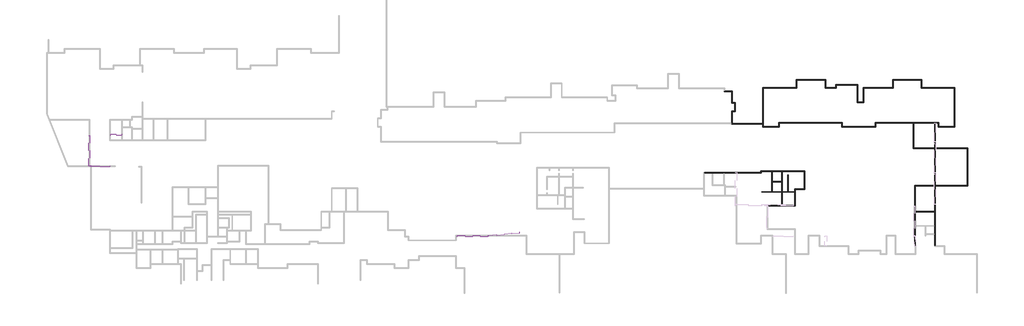
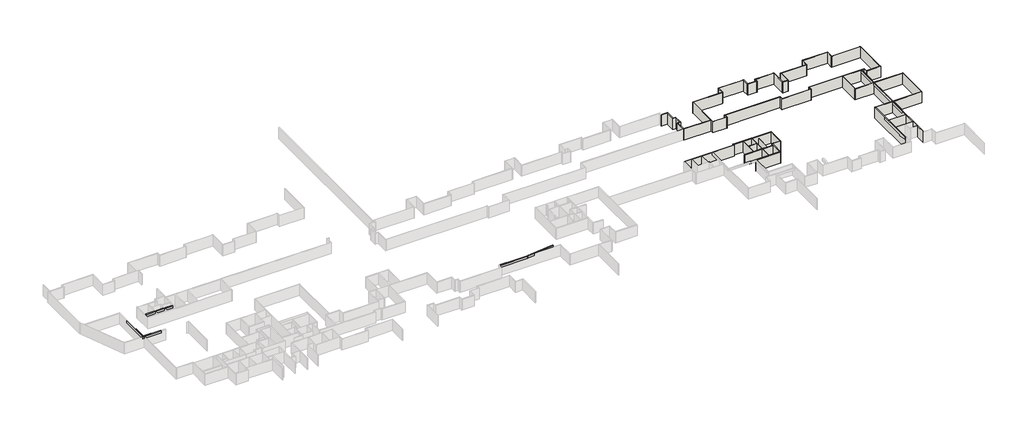
# One storey, part 7 of 8: 55 walls, 5 beams.
"""IFC4 building model written with IfcOpenShell, lengths in millimetres."""

from ifc_helpers import new_model, si_unit, frame, origin, origin_with_axes, place, context, project, spatial, polyline, outline, extrude, faceted_brep, element, save

model = new_model("IFC4")

# Units and contexts
model_context = context("Model", 3, world=origin())
ifc_project = project(units=[si_unit("LENGTHUNIT", "METRE", prefix="MILLI")], contexts=[model_context])

# Site, building, storey
site = spatial("IfcSite", under=ifc_project)
building = spatial("IfcBuilding", under=site)
storey = spatial("IfcBuildingStorey", under=building, Name="户型图", Elevation=0.0)

# Beams
placement = place(None, origin())
element("IfcBeam", 1, ObjectType="混凝土 - 矩形梁 : KL_beam", at=placement, inside=storey, context=model_context, shape_type="Brep", body=[
    faceted_brep([(96423.8477403, 45092.6668088, 3300.0), (96723.8477403, 45092.6668088, 3300.0), (96723.8477403, 45182.6668088, 3300.0), (96723.8477403, 52816.9449825, 3300.0), (96466.2302805, 52816.9449825, 3300.0), (96423.8477403, 52816.9449825, 3300.0), (96423.8477403, 45092.6668088, 2700.0), (96423.8477403, 52816.9449825, 2700.0), (96723.8477403, 45092.6668088, 2700.0), (96466.2302805, 52816.9449825, 2700.0), (96723.8477403, 52816.9449825, 2700.0), (96723.8477403, 45182.6668088, 2700.0)], [[[0, 1, 2, 3, 4, 5]], [[6, 0, 5, 7]], [[8, 6, 7, 9, 10, 11]], [[1, 8, 11, 10, 3, 2]], [[1, 0, 6, 8]], [[3, 10, 9, 7, 5, 4]]]),
])
element("IfcBeam", 2, ObjectType="混凝土 - 矩形梁 : KL_beam", at=placement, inside=storey, context=model_context, shape_type="Brep", body=[
    faceted_brep([(96423.8477403, 44972.6668088, 3300.0), (96423.8477403, 44882.6668088, 3300.0), (96858.261361, 44882.6668088, 3300.0), (96858.261361, 44972.6668088, 3300.0), (96423.8477403, 44882.6668088, 2700.0), (96423.8477403, 44972.6668088, 2700.0), (96858.261361, 44972.6668088, 2700.0), (96858.261361, 44882.6668088, 2700.0)], [[[0, 1, 2, 3]], [[4, 5, 6, 7]], [[1, 4, 7, 2]], [[4, 1, 0, 5]], [[5, 0, 3, 6]], [[3, 2, 7, 6]]]),
    faceted_brep([(101648.7128309, 45182.6668088, 3300.0), (101648.7128309, 45182.6668088, 2700.0), (96723.8477403, 45182.6668088, 2700.0), (96723.8477403, 45182.6668088, 3300.0), (101648.7128309, 44882.6668088, 3300.0), (101648.7128309, 44882.6668088, 2700.0), (96723.8477403, 45092.6668088, 2700.0), (96723.8477403, 45092.6668088, 3300.0), (96978.261361, 45092.6668088, 2700.0), (96978.261361, 45092.6668088, 3300.0), (96978.261361, 44882.6668088, 2700.0), (96978.261361, 44882.6668088, 3300.0), (96978.261361, 44972.6668088, 3300.0)], [[[0, 1, 2, 3]], [[0, 4, 5, 1]], [[3, 2, 6, 7]], [[8, 9, 7, 6]], [[9, 8, 10, 11, 12]], [[4, 0, 3, 7, 9, 12, 11]], [[1, 5, 10, 8, 6, 2]], [[5, 4, 11, 10]]]),
])
element("IfcBeam", 3, ObjectType="混凝土 - 矩形梁 : KL_beam", at=placement, inside=storey, context=model_context, shape_type="SweptSolid", body=[
    extrude(outline(polyline([(188793.7845861, 27383.0583741), (188793.7845861, 27683.0583741), (196393.7845861, 27683.0583741), (196393.7845861, 27536.9862623), (196385.7175673, 27383.0583741), (188793.7845861, 27383.0583741)])), frame((0.0, 0.0, 2700.0), z_axis=(0.0, 0.0, 1.0), x_axis=(1.0, 0.0, 0.0)), (0.0, 0.0, 1.0), 600.0),
])
element("IfcBeam", 4, ObjectType="混凝土 - 矩形梁 : KL_beam", at=placement, inside=storey, context=model_context, shape_type="Brep", body=[
    faceted_brep([(196693.7845861, 27529.1304858, 3300.0), (196686.9330908, 27398.3961679, 3300.0), (204278.3545725, 28263.2416532, 3300.0), (204280.088311, 28283.0583741, 3300.0), (204293.7845861, 28439.6075155, 3300.0), (204293.7845861, 28566.9400301, 3300.0), (196693.7845861, 27701.1172453, 3300.0), (196693.7845861, 27683.0583741, 3300.0), (196686.9330908, 27398.3961679, 2700.0), (204278.3545725, 28263.2416532, 2700.0), (196693.7845861, 27529.1304858, 2700.0), (196693.7845861, 27683.0583741, 2700.0), (196693.7845861, 27701.1172453, 2700.0), (204293.7845861, 28566.9400301, 2700.0), (204293.7845861, 28439.6075155, 2700.0), (204280.088311, 28283.0583741, 2700.0)], [[[0, 1, 2, 3, 4, 5, 6, 7]], [[1, 8, 9, 2]], [[8, 10, 11, 12, 13, 14, 15, 9]], [[12, 6, 5, 13]], [[6, 12, 11, 10, 0, 7]], [[1, 0, 10, 8]], [[5, 4, 14, 13]], [[2, 9, 15, 14, 4, 3]]]),
])
element("IfcBeam", 5, ObjectType="混凝土 - 矩形梁 : KL_beam", at=placement, inside=storey, context=model_context, shape_type="Brep", body=[
    faceted_brep([(109598.8477351, 52816.9449825, 3300.0), (109598.8477351, 53082.6668088, 3300.0), (109598.8477351, 53116.9449825, 3300.0), (107358.8477337, 53116.9449825, 3300.0), (107358.8477337, 52816.9449825, 3300.0), (109598.8477351, 52816.9449825, 2700.0), (107358.8477337, 52816.9449825, 2700.0), (109598.8477351, 53116.9449825, 2700.0), (109598.8477351, 53082.6668088, 2700.0), (107358.8477337, 53116.9449825, 2700.0)], [[[0, 1, 2, 3, 4]], [[5, 0, 4, 6]], [[7, 8, 5, 6, 9]], [[2, 7, 9, 3]], [[0, 5, 8, 7, 2, 1]], [[4, 3, 9, 6]]]),
    faceted_brep([(101948.7128309, 52816.9449825, 3300.0), (101948.7128309, 53116.9449825, 3300.0), (101948.7128309, 53116.9449825, 2700.0), (101948.7128309, 52816.9449825, 2700.0), (104655.6151291, 53116.9449825, 3300.0), (104655.6151291, 52816.9449825, 3300.0), (104655.6151291, 52816.9449825, 2700.0), (104655.6151291, 53116.9449825, 2700.0)], [[[0, 1, 2, 3]], [[4, 5, 6, 7]], [[1, 0, 5, 4]], [[0, 3, 6, 5]], [[3, 2, 7, 6]], [[2, 1, 4, 7]]]),
    faceted_brep([(104775.6151291, 52816.9449825, 3300.0), (104775.6151291, 53116.9449825, 3300.0), (104775.6151291, 53116.9449825, 2700.0), (104775.6151291, 52816.9449825, 2700.0), (107238.8477337, 53116.9449825, 3300.0), (107238.8477337, 52816.9449825, 3300.0), (107238.8477337, 52816.9449825, 2700.0), (107238.8477337, 53116.9449825, 2700.0)], [[[0, 1, 2, 3]], [[4, 5, 6, 7]], [[1, 0, 5, 4]], [[0, 3, 6, 5]], [[3, 2, 7, 6]], [[2, 1, 4, 7]]]),
])

# Walls
element("IfcWall", 6, ObjectType="所有墙体", at=placement, inside=storey, context=model_context, shape_type="Brep", body=[
    faceted_brep([(308483.5691593, 25066.2785565, 0.0), (308483.5691593, 40156.649759, 0.0), (308483.5691593, 40156.649759, 3300.0), (308483.5691593, 25066.2785565, 3300.0), (308363.5691593, 25066.2785565, 0.0), (308363.5691593, 25066.2785565, 3300.0), (308363.5691593, 27981.6313737, 3300.0), (308363.5691593, 28101.6313737, 3300.0), (308363.5691593, 30029.7325058, 3300.0), (308363.5691593, 30149.7325058, 3300.0), (308363.5691593, 33606.8475615, 3300.0), (308363.5691593, 33726.8475615, 3300.0), (308363.5691593, 40156.649759, 3300.0), (308363.5691593, 40156.649759, 0.0), (308363.5691593, 33726.8475615, 0.0), (308363.5691593, 33606.8475615, 0.0), (308363.5691593, 30149.7325058, 0.0), (308363.5691593, 30029.7325058, 0.0), (308363.5691593, 28101.6313737, 0.0), (308363.5691593, 27981.6313737, 0.0)], [[[0, 1, 2, 3]], [[4, 5, 6, 7, 8, 9, 10, 11, 12, 13, 14, 15, 16, 17, 18, 19]], [[1, 0, 4, 19, 18, 17, 16, 15, 14, 13]], [[3, 2, 12, 11, 10, 9, 8, 7, 6, 5]], [[0, 3, 5, 4]], [[2, 1, 13, 12]]]),
])
element("IfcWall", 7, ObjectType="所有墙体", at=placement, inside=storey, context=model_context, shape_type="Brep", body=[
    faceted_brep([(303458.8473874, 40156.649759, 0.0), (308363.5691593, 40156.649759, 0.0), (308483.5691593, 40156.649759, 0.0), (316708.8239545, 40156.649759, 0.0), (316708.8239545, 40156.649759, 3300.0), (308483.5691593, 40156.649759, 3300.0), (308363.5691593, 40156.649759, 3300.0), (303458.8473874, 40156.649759, 3300.0), (303458.8473874, 40276.649759, 0.0), (303458.8473874, 40276.649759, 3300.0), (308363.5691593, 40276.649759, 3300.0), (308483.5691593, 40276.649759, 3300.0), (316588.8239545, 40276.649759, 3300.0), (316708.8239545, 40276.649759, 3300.0), (316708.8239545, 40276.649759, 0.0), (316588.8239545, 40276.649759, 0.0), (308483.5691593, 40276.649759, 0.0), (308363.5691593, 40276.649759, 0.0)], [[[0, 1, 2, 3, 4, 5, 6, 7]], [[8, 9, 10, 11, 12, 13, 14, 15, 16, 17]], [[3, 2, 1, 0, 8, 17, 16, 15, 14]], [[7, 6, 5, 4, 13, 12, 11, 10, 9]], [[4, 3, 14, 13]], [[0, 7, 9, 8]]]),
])
element("IfcWall", 8, ObjectType="所有墙体", at=placement, inside=storey, context=model_context, shape_type="Brep", body=[
    faceted_brep([(316708.8239545, 40276.649759, 0.0), (316708.8239545, 49676.9053712, 0.0), (316708.8239545, 49676.9053712, 3300.0), (316708.8239545, 40276.649759, 3300.0), (316588.8239545, 40276.649759, 0.0), (316588.8239545, 40276.649759, 3300.0), (316588.8239545, 49556.9053712, 3300.0), (316588.8239545, 49676.9053712, 3300.0), (316588.8239545, 49676.9053712, 0.0), (316588.8239545, 49556.9053712, 0.0)], [[[0, 1, 2, 3]], [[4, 5, 6, 7, 8, 9]], [[1, 0, 4, 9, 8]], [[3, 2, 7, 6, 5]], [[0, 3, 5, 4]], [[2, 1, 8, 7]]]),
])
element("IfcWall", 9, ObjectType="所有墙体", at=placement, inside=storey, context=model_context, shape_type="SweptSolid", body=[
    extrude(outline(polyline([(308483.5691593, 49676.9053712), (316588.8239545, 49676.9053712), (316588.8239545, 49556.9053712), (308483.5691593, 49556.9053712), (308483.5691593, 49676.9053712)])), origin_with_axes(), (0.0, 0.0, 1.0), 3300.0),
])
element("IfcWall", 10, ObjectType="所有墙体", at=placement, inside=storey, context=model_context, shape_type="Brep", body=[
    faceted_brep([(308483.5691593, 40276.649759, 0.0), (308483.5691593, 49556.9053712, 0.0), (308483.5691593, 49676.9053712, 0.0), (308483.5691593, 55854.3583824, 0.0), (308483.5691593, 55854.3583824, 3300.0), (308483.5691593, 49676.9053712, 3300.0), (308483.5691593, 49556.9053712, 3300.0), (308483.5691593, 40276.649759, 3300.0), (308363.5691593, 40276.649759, 0.0), (308363.5691593, 40276.649759, 3300.0), (308363.5691593, 49556.9053712, 3300.0), (308363.5691593, 49676.9053712, 3300.0), (308363.5691593, 55854.3583824, 3300.0), (308363.5691593, 55854.3583824, 0.0), (308363.5691593, 49676.9053712, 0.0), (308363.5691593, 49556.9053712, 0.0)], [[[0, 1, 2, 3, 4, 5, 6, 7]], [[8, 9, 10, 11, 12, 13, 14, 15]], [[3, 2, 1, 0, 8, 15, 14, 13]], [[7, 6, 5, 4, 12, 11, 10, 9]], [[4, 3, 13, 12]], [[0, 7, 9, 8]]]),
])
element("IfcWall", 11, ObjectType="所有墙体", at=placement, inside=storey, context=model_context, shape_type="Brep", body=[
    faceted_brep([(293431.9735661, 55854.3583824, 0.0), (293551.9735661, 55854.3583824, 0.0), (302988.8797699, 55854.3583824, 0.0), (303108.8797699, 55854.3583824, 0.0), (308363.5691593, 55854.3583824, 0.0), (308483.5691593, 55854.3583824, 0.0), (309231.9735597, 55854.3583824, 0.0), (309351.9735597, 55854.3583824, 0.0), (309351.9735597, 55854.3583824, 3300.0), (309231.9735597, 55854.3583824, 3300.0), (308483.5691593, 55854.3583824, 3300.0), (308363.5691593, 55854.3583824, 3300.0), (303108.8797699, 55854.3583824, 3300.0), (302988.8797699, 55854.3583824, 3300.0), (293551.9735661, 55854.3583824, 3300.0), (293431.9735661, 55854.3583824, 3300.0), (293431.9735661, 55974.3583824, 0.0), (293431.9735661, 55974.3583824, 3300.0), (309351.9735597, 55974.3583824, 3300.0), (309351.9735597, 55974.3583824, 0.0)], [[[0, 1, 2, 3, 4, 5, 6, 7, 8, 9, 10, 11, 12, 13, 14, 15]], [[16, 17, 18, 19]], [[7, 6, 5, 4, 3, 2, 1, 0, 16, 19]], [[15, 14, 13, 12, 11, 10, 9, 8, 18, 17]], [[8, 7, 19, 18]], [[0, 15, 17, 16]]]),
])
element("IfcWall", 12, ObjectType="所有墙体", at=placement, inside=storey, context=model_context, shape_type="Brep", body=[
    faceted_brep([(309231.9735597, 55854.3583824, 0.0), (309231.9735597, 54854.3583848, 0.0), (309231.9735597, 54854.3583848, 3300.0), (309231.9735597, 55854.3583824, 3300.0), (309351.9735597, 55854.3583824, 0.0), (309351.9735597, 55854.3583824, 3300.0), (309351.9735597, 54974.3583848, 3300.0), (309351.9735597, 54854.3583848, 3300.0), (309351.9735597, 54854.3583848, 0.0), (309351.9735597, 54974.3583848, 0.0)], [[[0, 1, 2, 3]], [[4, 5, 6, 7, 8, 9]], [[1, 0, 4, 9, 8]], [[3, 2, 7, 6, 5]], [[0, 3, 5, 4]], [[2, 1, 8, 7]]]),
])
element("IfcWall", 13, ObjectType="所有墙体", at=placement, inside=storey, context=model_context, shape_type="Brep", body=[
    faceted_brep([(309351.9735597, 54854.3583848, 0.0), (313351.9735669, 54854.3583848, 0.0), (313351.9735669, 54854.3583848, 3300.0), (309351.9735597, 54854.3583848, 3300.0), (309351.9735597, 54974.3583848, 0.0), (309351.9735597, 54974.3583848, 3300.0), (313231.9735669, 54974.3583848, 3300.0), (313351.9735669, 54974.3583848, 3300.0), (313351.9735669, 54974.3583848, 0.0), (313231.9735669, 54974.3583848, 0.0)], [[[0, 1, 2, 3]], [[4, 5, 6, 7, 8, 9]], [[1, 0, 4, 9, 8]], [[3, 2, 7, 6, 5]], [[0, 3, 5, 4]], [[2, 1, 8, 7]]]),
])
element("IfcWall", 14, ObjectType="所有墙体", at=placement, inside=storey, context=model_context, shape_type="Brep", body=[
    faceted_brep([(313351.9735669, 54974.3583848, 0.0), (313351.9735669, 64774.3583829, 0.0), (313351.9735669, 64774.3583829, 3300.0), (313351.9735669, 54974.3583848, 3300.0), (313231.9735669, 54974.3583848, 0.0), (313231.9735669, 54974.3583848, 3300.0), (313231.9735669, 64654.3583829, 3300.0), (313231.9735669, 64774.3583829, 3300.0), (313231.9735669, 64774.3583829, 0.0), (313231.9735669, 64654.3583829, 0.0)], [[[0, 1, 2, 3]], [[4, 5, 6, 7, 8, 9]], [[1, 0, 4, 9, 8]], [[3, 2, 7, 6, 5]], [[0, 3, 5, 4]], [[2, 1, 8, 7]]]),
])
element("IfcWall", 15, ObjectType="所有墙体", at=placement, inside=storey, context=model_context, shape_type="Brep", body=[
    faceted_brep([(313231.9735669, 64774.3583829, 0.0), (305151.9735626, 64774.3583829, 0.0), (305031.9735626, 64774.3583829, 0.0), (305031.9735626, 64774.3583829, 3300.0), (305151.9735626, 64774.3583829, 3300.0), (313231.9735669, 64774.3583829, 3300.0), (313231.9735669, 64654.3583829, 0.0), (313231.9735669, 64654.3583829, 3300.0), (305031.9735626, 64654.3583829, 3300.0), (305031.9735626, 64654.3583829, 0.0)], [[[0, 1, 2, 3, 4, 5]], [[6, 7, 8, 9]], [[2, 1, 0, 6, 9]], [[5, 4, 3, 8, 7]], [[0, 5, 7, 6]], [[3, 2, 9, 8]]]),
])
element("IfcWall", 16, ObjectType="所有墙体", at=placement, inside=storey, context=model_context, shape_type="Brep", body=[
    faceted_brep([(305151.9735626, 64774.3583829, 0.0), (305151.9735626, 66774.3583864, 0.0), (305151.9735626, 66774.3583864, 3300.0), (305151.9735626, 64774.3583829, 3300.0), (305031.9735626, 64774.3583829, 0.0), (305031.9735626, 64774.3583829, 3300.0), (305031.9735626, 66654.3583864, 3300.0), (305031.9735626, 66774.3583864, 3300.0), (305031.9735626, 66774.3583864, 0.0), (305031.9735626, 66654.3583864, 0.0)], [[[0, 1, 2, 3]], [[4, 5, 6, 7, 8, 9]], [[1, 0, 4, 9, 8]], [[3, 2, 7, 6, 5]], [[0, 3, 5, 4]], [[2, 1, 8, 7]]]),
])
element("IfcWall", 17, ObjectType="所有墙体", at=placement, inside=storey, context=model_context, shape_type="Brep", body=[
    faceted_brep([(305031.9735626, 66774.3583864, 0.0), (297831.9735583, 66774.3583864, 0.0), (297831.9735583, 66774.3583864, 3300.0), (305031.9735626, 66774.3583864, 3300.0), (305031.9735626, 66654.3583864, 0.0), (305031.9735626, 66654.3583864, 3300.0), (297951.9735583, 66654.3583864, 3300.0), (297831.9735583, 66654.3583864, 3300.0), (297831.9735583, 66654.3583864, 0.0), (297951.9735583, 66654.3583864, 0.0)], [[[0, 1, 2, 3]], [[4, 5, 6, 7, 8, 9]], [[1, 0, 4, 9, 8]], [[3, 2, 7, 6, 5]], [[0, 3, 5, 4]], [[2, 1, 8, 7]]]),
])
element("IfcWall", 18, ObjectType="所有墙体", at=placement, inside=storey, context=model_context, shape_type="Brep", body=[
    faceted_brep([(297831.9735583, 66654.3583864, 0.0), (297831.9735583, 64774.3583829, 0.0), (297831.9735583, 64654.3583829, 0.0), (297831.9735583, 64654.3583829, 3300.0), (297831.9735583, 64774.3583829, 3300.0), (297831.9735583, 66654.3583864, 3300.0), (297951.9735583, 66654.3583864, 0.0), (297951.9735583, 66654.3583864, 3300.0), (297951.9735583, 64654.3583829, 3300.0), (297951.9735583, 64654.3583829, 0.0)], [[[0, 1, 2, 3, 4, 5]], [[6, 7, 8, 9]], [[2, 1, 0, 6, 9]], [[5, 4, 3, 8, 7]], [[0, 5, 7, 6]], [[3, 2, 9, 8]]]),
])
element("IfcWall", 19, ObjectType="所有墙体", at=placement, inside=storey, context=model_context, shape_type="Brep", body=[
    faceted_brep([(297831.9735583, 64774.3583829, 0.0), (290431.9735626, 64774.3583829, 0.0), (290431.9735626, 64774.3583829, 3300.0), (297831.9735583, 64774.3583829, 3300.0), (297831.9735583, 64654.3583829, 0.0), (297831.9735583, 64654.3583829, 3300.0), (290551.9735626, 64654.3583829, 3300.0), (290431.9735626, 64654.3583829, 3300.0), (290431.9735626, 64654.3583829, 0.0), (290551.9735626, 64654.3583829, 0.0)], [[[0, 1, 2, 3]], [[4, 5, 6, 7, 8, 9]], [[1, 0, 4, 9, 8]], [[3, 2, 7, 6, 5]], [[0, 3, 5, 4]], [[2, 1, 8, 7]]]),
])
element("IfcWall", 20, ObjectType="所有墙体", at=placement, inside=storey, context=model_context, shape_type="Brep", body=[
    faceted_brep([(290431.9735626, 64654.3583829, 0.0), (290431.9735626, 61174.3583823, 0.0), (290431.9735626, 61054.3583823, 0.0), (290431.9735626, 61054.3583823, 3300.0), (290431.9735626, 61174.3583823, 3300.0), (290431.9735626, 64654.3583829, 3300.0), (290551.9735626, 64654.3583829, 0.0), (290551.9735626, 64654.3583829, 3300.0), (290551.9735626, 61054.3583823, 3300.0), (290551.9735626, 61054.3583823, 0.0)], [[[0, 1, 2, 3, 4, 5]], [[6, 7, 8, 9]], [[2, 1, 0, 6, 9]], [[5, 4, 3, 8, 7]], [[0, 5, 7, 6]], [[3, 2, 9, 8]]]),
])
element("IfcWall", 21, ObjectType="所有墙体", at=placement, inside=storey, context=model_context, shape_type="Brep", body=[
    faceted_brep([(290431.9735626, 61174.3583823, 0.0), (289051.9735625, 61174.3583823, 0.0), (288931.9735625, 61174.3583823, 0.0), (288931.9735625, 61174.3583823, 3300.0), (289051.9735625, 61174.3583823, 3300.0), (290431.9735626, 61174.3583823, 3300.0), (290431.9735626, 61054.3583823, 0.0), (290431.9735626, 61054.3583823, 3300.0), (288931.9735625, 61054.3583823, 3300.0), (288931.9735625, 61054.3583823, 0.0)], [[[0, 1, 2, 3, 4, 5]], [[6, 7, 8, 9]], [[2, 1, 0, 6, 9]], [[5, 4, 3, 8, 7]], [[0, 5, 7, 6]], [[3, 2, 9, 8]]]),
])
element("IfcWall", 22, ObjectType="所有墙体", at=placement, inside=storey, context=model_context, shape_type="Brep", body=[
    faceted_brep([(289051.9735625, 61174.3583823, 0.0), (289051.9735625, 65574.3800091, 0.0), (289051.9735625, 65574.3800091, 3300.0), (289051.9735625, 61174.3583823, 3300.0), (288931.9735625, 61174.3583823, 0.0), (288931.9735625, 61174.3583823, 3300.0), (288931.9735625, 65454.3800091, 3300.0), (288931.9735625, 65574.3800091, 3300.0), (288931.9735625, 65574.3800091, 0.0), (288931.9735625, 65454.3800091, 0.0)], [[[0, 1, 2, 3]], [[4, 5, 6, 7, 8, 9]], [[1, 0, 4, 9, 8]], [[3, 2, 7, 6, 5]], [[0, 3, 5, 4]], [[2, 1, 8, 7]]]),
])
element("IfcWall", 23, ObjectType="所有墙体", at=placement, inside=storey, context=model_context, shape_type="Brep", body=[
    faceted_brep([(288931.9735625, 65574.3800091, 0.0), (283531.9735562, 65574.3800091, 0.0), (283531.9735562, 65574.3800091, 3300.0), (288931.9735625, 65574.3800091, 3300.0), (288931.9735625, 65454.3800091, 0.0), (288931.9735625, 65454.3800091, 3300.0), (283651.9735562, 65454.3800091, 3300.0), (283531.9735562, 65454.3800091, 3300.0), (283531.9735562, 65454.3800091, 0.0), (283651.9735562, 65454.3800091, 0.0)], [[[0, 1, 2, 3]], [[4, 5, 6, 7, 8, 9]], [[1, 0, 4, 9, 8]], [[3, 2, 7, 6, 5]], [[0, 3, 5, 4]], [[2, 1, 8, 7]]]),
])
element("IfcWall", 24, ObjectType="所有墙体", at=placement, inside=storey, context=model_context, shape_type="Brep", body=[
    faceted_brep([(283531.9735562, 65454.3800091, 0.0), (283531.9735562, 64774.3583829, 0.0), (283531.9735562, 64654.3583829, 0.0), (283531.9735562, 64654.3583829, 3300.0), (283531.9735562, 64774.3583829, 3300.0), (283531.9735562, 65454.3800091, 3300.0), (283651.9735562, 65454.3800091, 0.0), (283651.9735562, 65454.3800091, 3300.0), (283651.9735562, 64654.3583829, 3300.0), (283651.9735562, 64654.3583829, 0.0)], [[[0, 1, 2, 3, 4, 5]], [[6, 7, 8, 9]], [[2, 1, 0, 6, 9]], [[5, 4, 3, 8, 7]], [[0, 5, 7, 6]], [[3, 2, 9, 8]]]),
])
element("IfcWall", 25, ObjectType="所有墙体", at=placement, inside=storey, context=model_context, shape_type="Brep", body=[
    faceted_brep([(283531.9735562, 64774.3583829, 0.0), (281051.9735665, 64774.3583829, 0.0), (280931.9735665, 64774.3583829, 0.0), (280931.9735665, 64774.3583829, 3300.0), (281051.9735665, 64774.3583829, 3300.0), (283531.9735562, 64774.3583829, 3300.0), (283531.9735562, 64654.3583829, 0.0), (283531.9735562, 64654.3583829, 3300.0), (280931.9735665, 64654.3583829, 3300.0), (280931.9735665, 64654.3583829, 0.0)], [[[0, 1, 2, 3, 4, 5]], [[6, 7, 8, 9]], [[2, 1, 0, 6, 9]], [[5, 4, 3, 8, 7]], [[0, 5, 7, 6]], [[3, 2, 9, 8]]]),
])
element("IfcWall", 26, ObjectType="所有墙体", at=placement, inside=storey, context=model_context, shape_type="Brep", body=[
    faceted_brep([(281051.9735665, 64774.3583829, 0.0), (281051.9735665, 66774.3583864, 0.0), (281051.9735665, 66774.3583864, 3300.0), (281051.9735665, 64774.3583829, 3300.0), (280931.9735665, 64774.3583829, 0.0), (280931.9735665, 64774.3583829, 3300.0), (280931.9735665, 66654.3583864, 3300.0), (280931.9735665, 66774.3583864, 3300.0), (280931.9735665, 66774.3583864, 0.0), (280931.9735665, 66654.3583864, 0.0)], [[[0, 1, 2, 3]], [[4, 5, 6, 7, 8, 9]], [[1, 0, 4, 9, 8]], [[3, 2, 7, 6, 5]], [[0, 3, 5, 4]], [[2, 1, 8, 7]]]),
])
element("IfcWall", 27, ObjectType="所有墙体", at=placement, inside=storey, context=model_context, shape_type="Brep", body=[
    faceted_brep([(280931.9735665, 66774.3583864, 0.0), (273731.9735661, 66774.3583864, 0.0), (273731.9735661, 66774.3583864, 3300.0), (280931.9735665, 66774.3583864, 3300.0), (280931.9735665, 66654.3583864, 0.0), (280931.9735665, 66654.3583864, 3300.0), (273851.9735661, 66654.3583864, 3300.0), (273731.9735661, 66654.3583864, 3300.0), (273731.9735661, 66654.3583864, 0.0), (273851.9735661, 66654.3583864, 0.0)], [[[0, 1, 2, 3]], [[4, 5, 6, 7, 8, 9]], [[1, 0, 4, 9, 8]], [[3, 2, 7, 6, 5]], [[0, 3, 5, 4]], [[2, 1, 8, 7]]]),
])
element("IfcWall", 28, ObjectType="所有墙体", at=placement, inside=storey, context=model_context, shape_type="Brep", body=[
    faceted_brep([(273731.9735661, 66654.3583864, 0.0), (273731.9735661, 64774.3583829, 0.0), (273731.9735661, 64654.3583829, 0.0), (273731.9735661, 64654.3583829, 3300.0), (273731.9735661, 64774.3583829, 3300.0), (273731.9735661, 66654.3583864, 3300.0), (273851.9735661, 66654.3583864, 0.0), (273851.9735661, 66654.3583864, 3300.0), (273851.9735661, 64654.3583829, 3300.0), (273851.9735661, 64654.3583829, 0.0)], [[[0, 1, 2, 3, 4, 5]], [[6, 7, 8, 9]], [[2, 1, 0, 6, 9]], [[5, 4, 3, 8, 7]], [[0, 5, 7, 6]], [[3, 2, 9, 8]]]),
])
element("IfcWall", 29, ObjectType="所有墙体", at=placement, inside=storey, context=model_context, shape_type="Brep", body=[
    faceted_brep([(273731.9735661, 64774.3583829, 0.0), (265331.9735637, 64774.3583829, 0.0), (265331.9735637, 64774.3583829, 3300.0), (273731.9735661, 64774.3583829, 3300.0), (273731.9735661, 64654.3583829, 0.0), (273731.9735661, 64654.3583829, 3300.0), (265451.9735637, 64654.3583829, 3300.0), (265331.9735637, 64654.3583829, 3300.0), (265331.9735637, 64654.3583829, 0.0), (265451.9735637, 64654.3583829, 0.0)], [[[0, 1, 2, 3]], [[4, 5, 6, 7, 8, 9]], [[1, 0, 4, 9, 8]], [[3, 2, 7, 6, 5]], [[0, 3, 5, 4]], [[2, 1, 8, 7]]]),
])
element("IfcWall", 30, ObjectType="所有墙体", at=placement, inside=storey, context=model_context, shape_type="Brep", body=[
    faceted_brep([(265331.9735637, 64654.3583829, 0.0), (265331.9735637, 55826.5251182, 0.0), (265331.9735637, 55706.5251182, 0.0), (265331.9735637, 54974.3583848, 0.0), (265331.9735637, 54974.3583848, 3300.0), (265331.9735637, 55706.5251182, 3300.0), (265331.9735637, 55826.5251182, 3300.0), (265331.9735637, 64654.3583829, 3300.0), (265451.9735637, 64654.3583829, 0.0), (265451.9735637, 64654.3583829, 3300.0), (265451.9735637, 54974.3583848, 3300.0), (265451.9735637, 54974.3583848, 0.0)], [[[0, 1, 2, 3, 4, 5, 6, 7]], [[8, 9, 10, 11]], [[3, 2, 1, 0, 8, 11]], [[7, 6, 5, 4, 10, 9]], [[0, 7, 9, 8]], [[4, 3, 11, 10]]]),
])
element("IfcWall", 31, ObjectType="所有墙体", at=placement, inside=storey, context=model_context, shape_type="Brep", body=[
    faceted_brep([(265331.9735637, 55826.5251182, 0.0), (257584.5015155, 55826.5251182, 0.0), (257464.5015155, 55826.5251182, 0.0), (257464.5015155, 55826.5251182, 3300.0), (257584.5015155, 55826.5251182, 3300.0), (265331.9735637, 55826.5251182, 3300.0), (265331.9735637, 55706.5251182, 0.0), (265331.9735637, 55706.5251182, 3300.0), (257464.5015155, 55706.5251182, 3300.0), (257464.5015155, 55706.5251182, 0.0), (257464.5015155, 55756.5110329, 0.0), (257464.5015155, 55756.5110329, 3300.0)], [[[0, 1, 2, 3, 4, 5]], [[6, 7, 8, 9]], [[2, 1, 0, 6, 9, 10]], [[5, 4, 3, 11, 8, 7]], [[0, 5, 7, 6]], [[3, 2, 10, 9, 8, 11]]]),
])
element("IfcWall", 32, ObjectType="所有墙体", at=placement, inside=storey, context=model_context, shape_type="Brep", body=[
    faceted_brep([(257584.5015155, 55826.5251182, 0.0), (257584.5015155, 58756.6395115, 0.0), (257584.5015155, 58876.6395115, 0.0), (257584.5015155, 58876.6395115, 3300.0), (257584.5015155, 58756.6395115, 3300.0), (257584.5015155, 55826.5251182, 3300.0), (257464.5015155, 55826.5251182, 0.0), (257464.5015155, 55826.5251182, 3300.0), (257464.5015155, 55876.5110329, 3300.0), (257464.5015155, 58876.6395115, 3300.0), (257464.5015155, 58876.6395115, 0.0), (257464.5015155, 55876.5110329, 0.0)], [[[0, 1, 2, 3, 4, 5]], [[6, 7, 8, 9, 10, 11]], [[2, 1, 0, 6, 11, 10]], [[5, 4, 3, 9, 8, 7]], [[0, 5, 7, 6]], [[3, 2, 10, 9]]]),
])
element("IfcWall", 33, ObjectType="所有墙体", at=placement, inside=storey, context=model_context, shape_type="Brep", body=[
    faceted_brep([(257584.5015155, 58756.6395115, 0.0), (258384.5015175, 58756.6395115, 0.0), (258384.5015175, 58756.6395115, 3300.0), (257584.5015155, 58756.6395115, 3300.0), (257584.5015155, 58876.6395115, 0.0), (257584.5015155, 58876.6395115, 3300.0), (258264.5015175, 58876.6395115, 3300.0), (258384.5015175, 58876.6395115, 3300.0), (258384.5015175, 58876.6395115, 0.0), (258264.5015175, 58876.6395115, 0.0)], [[[0, 1, 2, 3]], [[4, 5, 6, 7, 8, 9]], [[1, 0, 4, 9, 8]], [[3, 2, 7, 6, 5]], [[0, 3, 5, 4]], [[2, 1, 8, 7]]]),
])
element("IfcWall", 34, ObjectType="所有墙体", at=placement, inside=storey, context=model_context, shape_type="Brep", body=[
    faceted_brep([(258384.5015175, 58876.6395115, 0.0), (258384.5015175, 61076.6395927, 0.0), (258384.5015175, 61076.6395927, 3300.0), (258384.5015175, 58876.6395115, 3300.0), (258264.5015175, 58876.6395115, 0.0), (258264.5015175, 58876.6395115, 3300.0), (258264.5015175, 60956.6395927, 3300.0), (258264.5015175, 61076.6395927, 3300.0), (258264.5015175, 61076.6395927, 0.0), (258264.5015175, 60956.6395927, 0.0)], [[[0, 1, 2, 3]], [[4, 5, 6, 7, 8, 9]], [[1, 0, 4, 9, 8]], [[3, 2, 7, 6, 5]], [[0, 3, 5, 4]], [[2, 1, 8, 7]]]),
])
element("IfcWall", 35, ObjectType="所有墙体", at=placement, inside=storey, context=model_context, shape_type="Brep", body=[
    faceted_brep([(258264.5015175, 61076.6395927, 0.0), (257584.5015155, 61076.6395927, 0.0), (257464.5015155, 61076.6395927, 0.0), (257464.5015155, 61076.6395927, 3300.0), (257584.5015155, 61076.6395927, 3300.0), (258264.5015175, 61076.6395927, 3300.0), (258264.5015175, 60956.6395927, 0.0), (258264.5015175, 60956.6395927, 3300.0), (257464.5015155, 60956.6395927, 3300.0), (257464.5015155, 60956.6395927, 0.0)], [[[0, 1, 2, 3, 4, 5]], [[6, 7, 8, 9]], [[2, 1, 0, 6, 9]], [[5, 4, 3, 8, 7]], [[0, 5, 7, 6]], [[3, 2, 9, 8]]]),
])
element("IfcWall", 36, ObjectType="所有墙体", at=placement, inside=storey, context=model_context, shape_type="Brep", body=[
    faceted_brep([(257584.5015155, 61076.6395927, 0.0), (257584.5015155, 63876.5127734, 0.0), (257584.5015155, 63876.5127734, 3300.0), (257584.5015155, 61076.6395927, 3300.0), (257464.5015155, 61076.6395927, 0.0), (257464.5015155, 61076.6395927, 3300.0), (257464.5015155, 63756.5127734, 3300.0), (257464.5015155, 63876.5127734, 3300.0), (257464.5015155, 63876.5127734, 0.0), (257464.5015155, 63756.5127734, 0.0)], [[[0, 1, 2, 3]], [[4, 5, 6, 7, 8, 9]], [[1, 0, 4, 9, 8]], [[3, 2, 7, 6, 5]], [[0, 3, 5, 4]], [[2, 1, 8, 7]]]),
])
element("IfcWall", 37, ObjectType="所有墙体", at=placement, inside=storey, context=model_context, shape_type="Brep", body=[
    faceted_brep([(257464.5015155, 63876.5127734, 0.0), (255784.4931741, 63876.5127734, 0.0), (255664.4931741, 63876.5127734, 0.0), (255664.4931741, 63876.5127734, 3300.0), (255784.4931741, 63876.5127734, 3300.0), (257464.5015155, 63876.5127734, 3300.0), (257464.5015155, 63756.5127734, 0.0), (257464.5015155, 63756.5127734, 3300.0), (255664.4931741, 63756.5127734, 3300.0), (255664.4931741, 63756.5127734, 0.0)], [[[0, 1, 2, 3, 4, 5]], [[6, 7, 8, 9]], [[2, 1, 0, 6, 9]], [[5, 4, 3, 8, 7]], [[0, 5, 7, 6]], [[3, 2, 9, 8]]]),
])
element("IfcWall", 38, ObjectType="所有墙体", at=placement, inside=storey, context=model_context, shape_type="Brep", body=[
    faceted_brep([(250658.8239575, 43406.8473728, 0.0), (255513.6576827, 43406.8473728, 0.0), (255633.6576827, 43406.8473728, 0.0), (264932.3033606, 43406.8473728, 0.0), (264932.3033606, 43406.8473728, 3300.0), (255633.6576827, 43406.8473728, 3300.0), (255513.6576827, 43406.8473728, 3300.0), (250658.8239575, 43406.8473728, 3300.0), (250658.8239575, 43526.8473728, 0.0), (250658.8239575, 43526.8473728, 3300.0), (264812.3033606, 43526.8473728, 3300.0), (264932.3033606, 43526.8473728, 3300.0), (264932.3033606, 43526.8473728, 0.0), (264812.3033606, 43526.8473728, 0.0)], [[[0, 1, 2, 3, 4, 5, 6, 7]], [[8, 9, 10, 11, 12, 13]], [[3, 2, 1, 0, 8, 13, 12]], [[7, 6, 5, 4, 11, 10, 9]], [[0, 7, 9, 8]], [[4, 3, 12, 11]]]),
])
element("IfcWall", 39, ObjectType="所有墙体", at=placement, inside=storey, context=model_context, shape_type="Brep", body=[
    faceted_brep([(264932.3033606, 43526.8473728, 0.0), (264932.3033606, 43807.0754503, 0.0), (264932.3033606, 43927.0754503, 0.0), (264932.3033606, 43927.0754503, 3300.0), (264932.3033606, 43807.0754503, 3300.0), (264932.3033606, 43526.8473728, 3300.0), (264812.3033606, 43526.8473728, 0.0), (264812.3033606, 43526.8473728, 3300.0), (264812.3033606, 43927.0754503, 3300.0), (264812.3033606, 43927.0754503, 0.0)], [[[0, 1, 2, 3, 4, 5]], [[6, 7, 8, 9]], [[2, 1, 0, 6, 9]], [[5, 4, 3, 8, 7]], [[0, 5, 7, 6]], [[3, 2, 9, 8]]]),
])
element("IfcWall", 40, ObjectType="所有墙体", at=placement, inside=storey, context=model_context, shape_type="Brep", body=[
    faceted_brep([(264932.3033606, 43807.0754503, 0.0), (275663.8471108, 43807.0754503, 0.0), (275783.8471108, 43807.0754503, 0.0), (275783.8471108, 43807.0754503, 3300.0), (275663.8471108, 43807.0754503, 3300.0), (264932.3033606, 43807.0754503, 3300.0), (264932.3033606, 43927.0754503, 0.0), (264932.3033606, 43927.0754503, 3300.0), (275783.8471108, 43927.0754503, 3300.0), (275783.8471108, 43927.0754503, 0.0)], [[[0, 1, 2, 3, 4, 5]], [[6, 7, 8, 9]], [[2, 1, 0, 6, 9]], [[5, 4, 3, 8, 7]], [[0, 5, 7, 6]], [[3, 2, 9, 8]]]),
])
element("IfcWall", 41, ObjectType="所有墙体", at=placement, inside=storey, context=model_context, shape_type="Brep", body=[
    faceted_brep([(275663.8471108, 43807.0754503, 0.0), (275663.8471108, 39327.0768266, 0.0), (275663.8471108, 39207.0768266, 0.0), (275663.8471108, 39207.0768266, 3300.0), (275663.8471108, 39327.0768266, 3300.0), (275663.8471108, 43807.0754503, 3300.0), (275783.8471108, 43807.0754503, 0.0), (275783.8471108, 43807.0754503, 3300.0), (275783.8471108, 39207.0768266, 3300.0), (275783.8471108, 39207.0768266, 0.0)], [[[0, 1, 2, 3, 4, 5]], [[6, 7, 8, 9]], [[2, 1, 0, 6, 9]], [[5, 4, 3, 8, 7]], [[0, 5, 7, 6]], [[3, 2, 9, 8]]]),
])
element("IfcWall", 42, ObjectType="所有墙体", at=placement, inside=storey, context=model_context, shape_type="Brep", body=[
    faceted_brep([(275663.8471108, 39327.0768266, 0.0), (273288.1652502, 39327.0768266, 0.0), (273288.1652502, 39327.0768266, 3300.0), (275663.8471108, 39327.0768266, 3300.0), (275663.8471108, 39207.0768266, 0.0), (275663.8471108, 39207.0768266, 3300.0), (273408.1652502, 39207.0768266, 3300.0), (273288.1652502, 39207.0768266, 3300.0), (273288.1652502, 39207.0768266, 0.0), (273408.1652502, 39207.0768266, 0.0)], [[[0, 1, 2, 3]], [[4, 5, 6, 7, 8, 9]], [[1, 0, 4, 9, 8]], [[3, 2, 7, 6, 5]], [[0, 3, 5, 4]], [[2, 1, 8, 7]]]),
])
element("IfcWall", 43, ObjectType="所有墙体", at=placement, inside=storey, context=model_context, shape_type="Brep", body=[
    faceted_brep([(273288.1652502, 39207.0768266, 0.0), (273288.1652502, 35226.5508771, 0.0), (273288.1652502, 35106.5508771, 0.0), (273288.1652502, 35106.5508771, 3300.0), (273288.1652502, 35226.5508771, 3300.0), (273288.1652502, 39207.0768266, 3300.0), (273408.1652502, 39207.0768266, 0.0), (273408.1652502, 39207.0768266, 3300.0), (273408.1652502, 35106.5508771, 3300.0), (273408.1652502, 35106.5508771, 0.0)], [[[0, 1, 2, 3, 4, 5]], [[6, 7, 8, 9]], [[2, 1, 0, 6, 9]], [[5, 4, 3, 8, 7]], [[0, 5, 7, 6]], [[3, 2, 9, 8]]]),
])
element("IfcWall", 44, ObjectType="所有墙体", at=placement, inside=storey, context=model_context, shape_type="Brep", body=[
    faceted_brep([(273288.1652502, 35226.5508771, 0.0), (266363.353082, 35226.5508771, 0.0), (266363.353082, 35226.5508771, 3300.0), (273288.1652502, 35226.5508771, 3300.0), (273288.1652502, 35106.5508771, 0.0), (273288.1652502, 35106.5508771, 3300.0), (266483.353082, 35106.5508771, 3300.0), (266363.353082, 35106.5508771, 3300.0), (266363.353082, 35106.5508771, 0.0), (266483.353082, 35106.5508771, 0.0)], [[[0, 1, 2, 3]], [[4, 5, 6, 7, 8, 9]], [[1, 0, 4, 9, 8]], [[3, 2, 7, 6, 5]], [[0, 3, 5, 4]], [[2, 1, 8, 7]]]),
])
element("IfcWall", 45, ObjectType="所有墙体", at=placement, inside=storey, context=model_context, shape_type="Brep", body=[
    faceted_brep([(303458.8473874, 25067.4234213, 0.0), (303458.8473874, 30029.7325058, 0.0), (303458.8473874, 30149.7325058, 0.0), (303458.8473874, 33606.8475615, 0.0), (303458.8473874, 33726.8475615, 0.0), (303458.8473874, 40156.649759, 0.0), (303458.8473874, 40276.649759, 0.0), (303458.8473874, 40276.649759, 3300.0), (303458.8473874, 40156.649759, 3300.0), (303458.8473874, 33726.8475615, 3300.0), (303458.8473874, 33606.8475615, 3300.0), (303458.8473874, 30149.7325058, 3300.0), (303458.8473874, 30029.7325058, 3300.0), (303458.8473874, 25067.4234213, 3300.0), (303338.8473874, 25067.4234213, 0.0), (303338.8473874, 25067.4234213, 3300.0), (303338.8473874, 40276.649759, 3300.0), (303338.8473874, 40276.649759, 0.0)], [[[0, 1, 2, 3, 4, 5, 6, 7, 8, 9, 10, 11, 12, 13]], [[14, 15, 16, 17]], [[6, 5, 4, 3, 2, 1, 0, 14, 17]], [[13, 12, 11, 10, 9, 8, 7, 16, 15]], [[0, 13, 15, 14]], [[7, 6, 17, 16]]]),
])
element("IfcWall", 46, ObjectType="所有墙体", at=placement, inside=storey, context=model_context, shape_type="Brep", body=[
    faceted_brep([(308363.5691593, 49676.9053712, 0.0), (303108.8797699, 49676.9053712, 0.0), (302988.8797699, 49676.9053712, 0.0), (302988.8797699, 49676.9053712, 3300.0), (303108.8797699, 49676.9053712, 3300.0), (308363.5691593, 49676.9053712, 3300.0), (308363.5691593, 49556.9053712, 0.0), (308363.5691593, 49556.9053712, 3300.0), (302988.8797699, 49556.9053712, 3300.0), (302988.8797699, 49556.9053712, 0.0)], [[[0, 1, 2, 3, 4, 5]], [[6, 7, 8, 9]], [[2, 1, 0, 6, 9]], [[5, 4, 3, 8, 7]], [[0, 5, 7, 6]], [[3, 2, 9, 8]]]),
])
element("IfcWall", 47, ObjectType="所有墙体", at=placement, inside=storey, context=model_context, shape_type="SweptSolid", body=[
    extrude(outline(polyline([(303108.8797699, 55854.3583824), (303108.8797699, 49676.9053712), (302988.8797699, 49676.9053712), (302988.8797699, 55854.3583824), (303108.8797699, 55854.3583824)])), origin_with_axes(), (0.0, 0.0, 1.0), 3300.0),
])
element("IfcWall", 48, ObjectType="所有墙体", at=placement, inside=storey, context=model_context, shape_type="Brep", body=[
    faceted_brep([(293431.9735661, 55854.3583824, 0.0), (293431.9735661, 54974.3583848, 0.0), (293431.9735661, 54854.3583848, 0.0), (293431.9735661, 54854.3583848, 3300.0), (293431.9735661, 54974.3583848, 3300.0), (293431.9735661, 55854.3583824, 3300.0), (293551.9735661, 55854.3583824, 0.0), (293551.9735661, 55854.3583824, 3300.0), (293551.9735661, 54854.3583848, 3300.0), (293551.9735661, 54854.3583848, 0.0)], [[[0, 1, 2, 3, 4, 5]], [[6, 7, 8, 9]], [[2, 1, 0, 6, 9]], [[5, 4, 3, 8, 7]], [[0, 5, 7, 6]], [[3, 2, 9, 8]]]),
])
element("IfcWall", 49, ObjectType="所有墙体", at=placement, inside=storey, context=model_context, shape_type="Brep", body=[
    faceted_brep([(293431.9735661, 54974.3583848, 0.0), (285251.9735635, 54974.3583848, 0.0), (285131.9735635, 54974.3583848, 0.0), (285131.9735635, 54974.3583848, 3300.0), (285251.9735635, 54974.3583848, 3300.0), (293431.9735661, 54974.3583848, 3300.0), (293431.9735661, 54854.3583848, 0.0), (293431.9735661, 54854.3583848, 3300.0), (285131.9735635, 54854.3583848, 3300.0), (285131.9735635, 54854.3583848, 0.0)], [[[0, 1, 2, 3, 4, 5]], [[6, 7, 8, 9]], [[2, 1, 0, 6, 9]], [[5, 4, 3, 8, 7]], [[0, 5, 7, 6]], [[3, 2, 9, 8]]]),
])
element("IfcWall", 50, ObjectType="所有墙体", at=placement, inside=storey, context=model_context, shape_type="Brep", body=[
    faceted_brep([(285251.9735635, 54974.3583848, 0.0), (285251.9735635, 55974.3583824, 0.0), (285251.9735635, 55974.3583824, 3300.0), (285251.9735635, 54974.3583848, 3300.0), (285131.9735635, 54974.3583848, 0.0), (285131.9735635, 54974.3583848, 3300.0), (285131.9735635, 55854.3583824, 3300.0), (285131.9735635, 55974.3583824, 3300.0), (285131.9735635, 55974.3583824, 0.0), (285131.9735635, 55854.3583824, 0.0)], [[[0, 1, 2, 3]], [[4, 5, 6, 7, 8, 9]], [[1, 0, 4, 9, 8]], [[3, 2, 7, 6, 5]], [[0, 3, 5, 4]], [[2, 1, 8, 7]]]),
])
element("IfcWall", 51, ObjectType="所有墙体", at=placement, inside=storey, context=model_context, shape_type="Brep", body=[
    faceted_brep([(285131.9735635, 55974.3583824, 0.0), (269331.9735661, 55974.3583824, 0.0), (269331.9735661, 55974.3583824, 3300.0), (285131.9735635, 55974.3583824, 3300.0), (285131.9735635, 55854.3583824, 0.0), (285131.9735635, 55854.3583824, 3300.0), (269451.9735661, 55854.3583824, 3300.0), (269331.9735661, 55854.3583824, 3300.0), (269331.9735661, 55854.3583824, 0.0), (269451.9735661, 55854.3583824, 0.0)], [[[0, 1, 2, 3]], [[4, 5, 6, 7, 8, 9]], [[1, 0, 4, 9, 8]], [[3, 2, 7, 6, 5]], [[0, 3, 5, 4]], [[2, 1, 8, 7]]]),
])
element("IfcWall", 52, ObjectType="所有墙体", at=placement, inside=storey, context=model_context, shape_type="Brep", body=[
    faceted_brep([(269331.9735661, 55854.3583824, 0.0), (269331.9735661, 54974.3583848, 0.0), (269331.9735661, 54854.3583848, 0.0), (269331.9735661, 54854.3583848, 3300.0), (269331.9735661, 54974.3583848, 3300.0), (269331.9735661, 55854.3583824, 3300.0), (269451.9735661, 55854.3583824, 0.0), (269451.9735661, 55854.3583824, 3300.0), (269451.9735661, 54854.3583848, 3300.0), (269451.9735661, 54854.3583848, 0.0)], [[[0, 1, 2, 3, 4, 5]], [[6, 7, 8, 9]], [[2, 1, 0, 6, 9]], [[5, 4, 3, 8, 7]], [[0, 5, 7, 6]], [[3, 2, 9, 8]]]),
])
element("IfcWall", 53, ObjectType="所有墙体", at=placement, inside=storey, context=model_context, shape_type="Brep", body=[
    faceted_brep([(269331.9735661, 54974.3583848, 0.0), (265451.9735637, 54974.3583848, 0.0), (265331.9735637, 54974.3583848, 0.0), (265331.9735637, 54974.3583848, 3300.0), (265451.9735637, 54974.3583848, 3300.0), (269331.9735661, 54974.3583848, 3300.0), (269331.9735661, 54854.3583848, 0.0), (269331.9735661, 54854.3583848, 3300.0), (265331.9735637, 54854.3583848, 3300.0), (265331.9735637, 54854.3583848, 0.0)], [[[0, 1, 2, 3, 4, 5]], [[6, 7, 8, 9]], [[2, 1, 0, 6, 9]], [[5, 4, 3, 8, 7]], [[0, 5, 7, 6]], [[3, 2, 9, 8]]]),
])
element("IfcWall", 54, ObjectType="所有墙体", at=placement, inside=storey, context=model_context, shape_type="Brep", body=[
    faceted_brep([(265023.3530817, 38547.0768266, 0.0), (270038.1986789, 38547.0768266, 0.0), (270158.1986789, 38547.0768266, 0.0), (273084.4881621, 38547.0768266, 0.0), (273084.4881621, 38547.0768266, 3300.0), (270158.1986789, 38547.0768266, 3300.0), (270038.1986789, 38547.0768266, 3300.0), (265023.3530817, 38547.0768266, 3300.0), (265023.3530817, 38667.0768266, 0.0), (265023.3530817, 38667.0768266, 3300.0), (267563.3216388, 38667.0768266, 3300.0), (267683.3216388, 38667.0768266, 3300.0), (270038.1986789, 38667.0768266, 3300.0), (270158.1986789, 38667.0768266, 3300.0), (271513.3216538, 38667.0768266, 3300.0), (271633.3216538, 38667.0768266, 3300.0), (273084.4881621, 38667.0768266, 3300.0), (273084.4881621, 38667.0768266, 0.0), (271633.3216538, 38667.0768266, 0.0), (271513.3216538, 38667.0768266, 0.0), (270158.1986789, 38667.0768266, 0.0), (270038.1986789, 38667.0768266, 0.0), (267683.3216388, 38667.0768266, 0.0), (267563.3216388, 38667.0768266, 0.0)], [[[0, 1, 2, 3, 4, 5, 6, 7]], [[8, 9, 10, 11, 12, 13, 14, 15, 16, 17, 18, 19, 20, 21, 22, 23]], [[3, 2, 1, 0, 8, 23, 22, 21, 20, 19, 18, 17]], [[4, 3, 17, 16]], [[7, 6, 5, 4, 16, 15, 14, 13, 12, 11, 10, 9]], [[0, 7, 9, 8]]]),
])
element("IfcWall", 55, ObjectType="所有墙体", at=placement, inside=storey, context=model_context, shape_type="Brep", body=[
    faceted_brep([(267683.3216388, 38667.0768266, 0.0), (267683.3216388, 41157.0768113, 0.0), (267683.3216388, 41277.0768113, 0.0), (267683.3216388, 43647.0798304, 0.0), (267683.3216388, 43647.0798304, 3300.0), (267683.3216388, 41277.0768113, 3300.0), (267683.3216388, 41157.0768113, 3300.0), (267683.3216388, 38667.0768266, 3300.0), (267563.3216388, 38667.0768266, 0.0), (267563.3216388, 38667.0768266, 3300.0), (267563.3216388, 43647.0798304, 3300.0), (267563.3216388, 43647.0798304, 0.0)], [[[0, 1, 2, 3, 4, 5, 6, 7]], [[8, 9, 10, 11]], [[3, 2, 1, 0, 8, 11]], [[4, 3, 11, 10]], [[7, 6, 5, 4, 10, 9]], [[0, 7, 9, 8]]]),
])
element("IfcWall", 56, ObjectType="所有墙体", at=placement, inside=storey, context=model_context, shape_type="Brep", body=[
    faceted_brep([(270158.1986789, 38667.0768266, 0.0), (270158.1986789, 43647.0798304, 0.0), (270158.1986789, 43647.0798304, 3300.0), (270158.1986789, 38667.0768266, 3300.0), (270038.1986789, 38667.0768266, 0.0), (270038.1986789, 38667.0768266, 3300.0), (270038.1986789, 41157.0768113, 3300.0), (270038.1986789, 41277.0768113, 3300.0), (270038.1986789, 43647.0798304, 3300.0), (270038.1986789, 43647.0798304, 0.0), (270038.1986789, 41277.0768113, 0.0), (270038.1986789, 41157.0768113, 0.0)], [[[0, 1, 2, 3]], [[4, 5, 6, 7, 8, 9, 10, 11]], [[1, 0, 4, 11, 10, 9]], [[2, 1, 9, 8]], [[3, 2, 8, 7, 6, 5]], [[0, 3, 5, 4]]]),
])
element("IfcWall", 57, ObjectType="所有墙体", at=placement, inside=storey, context=model_context, shape_type="SweptSolid", body=[
    extrude(outline(polyline([(270038.1986789, 41157.0768113), (267683.3216388, 41157.0768113), (267683.3216388, 41277.0768113), (270038.1986789, 41277.0768113), (270038.1986789, 41157.0768113)])), origin_with_axes(), (0.0, 0.0, 1.0), 3300.0),
])
element("IfcWall", 58, ObjectType="所有墙体", at=placement, inside=storey, context=model_context, shape_type="SweptSolid", body=[
    extrude(outline(polyline([(271633.3216538, 42817.0764747), (271633.3216538, 38667.0768266), (271513.3216538, 38667.0768266), (271513.3216538, 42817.0764747), (271633.3216538, 42817.0764747)])), origin_with_axes(), (0.0, 0.0, 1.0), 3300.0),
])
element("IfcWall", 59, ObjectType="所有墙体", at=placement, inside=storey, context=model_context, shape_type="SweptSolid", body=[
    extrude(outline(polyline([(270038.1986789, 35291.452007), (270038.1986789, 38547.0768266), (270158.1986789, 38547.0768266), (270158.1986789, 35291.452007), (270038.1986789, 35291.452007)])), origin_with_axes(), (0.0, 0.0, 1.0), 3300.0),
])
element("IfcWall", 60, ObjectType="所有墙体", at=placement, inside=storey, context=model_context, shape_type="SweptSolid", body=[
    extrude(outline(polyline([(308363.5691593, 33606.8475615), (303458.8473874, 33606.8475615), (303458.8473874, 33726.8475615), (308363.5691593, 33726.8475615), (308363.5691593, 33606.8475615)])), origin_with_axes(), (0.0, 0.0, 1.0), 3300.0),
])

save(model, "model.ifc")

# Revit data of these elements
# Type "混凝土 - 矩形梁 : KL_beam"
#   Length [instance default] = 1524 mm
#   b = 300 mm
#   h = 600 mm
#   Structural Material [instance default] = 混凝土 - 现场浇注混凝土
#   Assembly Code = ""
# Type "所有墙体"
#   Layers, outside or top first: 120 mm "默认" (function 1)
# Elements 1, 2, 3, 4, 5 (IfcBeam, "混凝土 - 矩形梁 : KL_beam")
#   Comments = ""
#   Structural Material = none
#   Phase Created = 新构造
# Elements 6, 7, 8, 9, 10, 11, 12, 13, 14, 15, 16, 17, 18, 19, 20, 21, 22, 23, 24, 25, 26, 27, 28, 29, 30, 31, 32, 33, 34, 35, 36, 37, 38, 39, 40, 41, 42, 43, 44, 45, 46, 47, 48, 49, 50, 51, 52, 53, 54, 55, 56, 57, 58, 59, 60 (IfcWall, "所有墙体")
#   Top Offset = 0 mm
#   Base Offset = 0 mm
#   wall height = 3300 mm
#   Phase Created = 新构造
#   Base Constraint = 户型图
#   Top Constraint = 层高
#   Materials on its faces: "默认"
# Materials
#   "混凝土 - 现场浇注混凝土": class "混凝土", colour RGB 192 192 192, transparency 0
#   "默认": class "其他", colour RGB 192 192 192, transparency 0, Cost = 0
